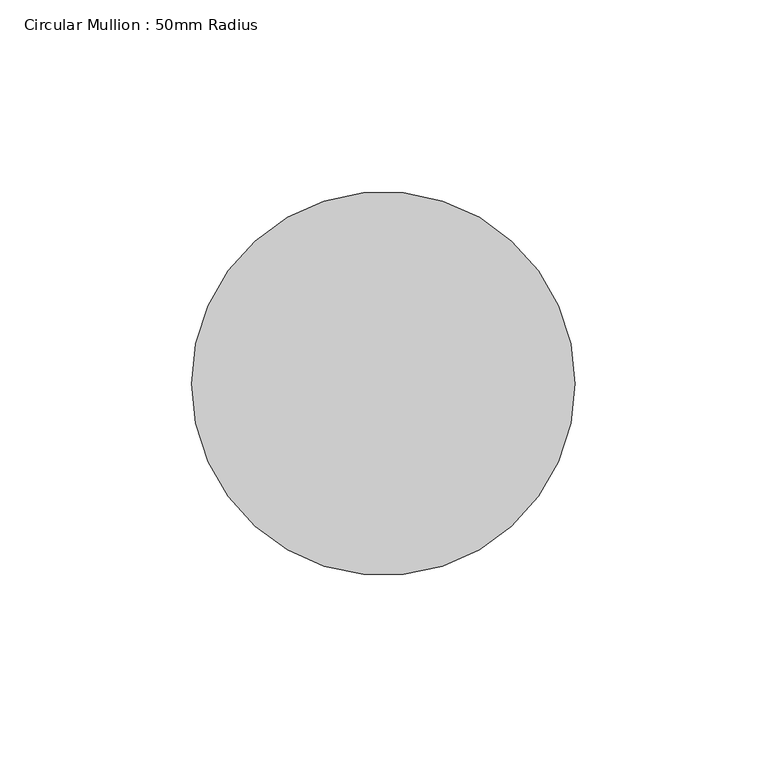
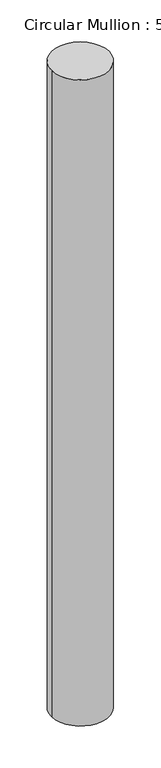
"""IFC4 building model written with IfcOpenShell, lengths in millimetres: member geometry, Circular Mullion : 50mm Radius."""

from ifc_helpers import new_model, si_unit, point, frame, origin, origin_2d, place, context, project, spatial, circle_curve, trimmed, segment, composite_curve, outline, extrude, source, transform, mapped, element, save


def circular_mullion_50mm_radius_da3aa2d7(model_context):
    return source(origin(), model_context, "Body", "SweptSolid", [
        extrude(outline(composite_curve([segment(trimmed(circle_curve(origin_2d(), 50.0), [point((50.0, 0.0))], [point((-50.0, 0.0))], False, "CARTESIAN"), True, "CONTINUOUS"), segment(trimmed(circle_curve(origin_2d(), 50.0), [point((-50.0, 0.0))], [point((50.0, 0.0))], False, "CARTESIAN"), True, "CONTINUOUS")], self_intersect=False)), frame((0.0, 0.0, -1186.6937644), z_axis=(0.0, 0.0, 1.0), x_axis=(1.0, 0.0, 0.0)), (0.0, 0.0, 1.0), 1186.6937644),
    ])


if __name__ == "__main__":
    model = new_model("IFC4")
    model_context = context("Model", 3, world=origin())
    ifc_project = project(units=[si_unit("LENGTHUNIT", "METRE", prefix="MILLI")], contexts=[model_context])
    site = spatial("IfcSite", under=ifc_project)
    building = spatial("IfcBuilding", under=site)
    placement = place(None, origin())
    circular_mullion_50mm_radius_shape = circular_mullion_50mm_radius_da3aa2d7(model_context)
    element("IfcMember", 1, ObjectType="Circular Mullion : 50mm Radius", at=placement, inside=building, context=model_context, shape_type="MappedRepresentation", body=[
        mapped(circular_mullion_50mm_radius_shape, transform((0.0, 0.0, 0.0), x_axis=(1.0, 0.0, 0.0), y_axis=(0.0, 1.0, 0.0), z_axis=(0.0, 0.0, 1.0))),
    ])
    save(model, "model.ifc")

# Revit data of these elements
# Type "Circular Mullion : 50mm Radius"
#   built-in parameter 1007350 = 0.164042 (stored number, unit not read)
# Element 1 (IfcMember, "Circular Mullion : 50mm Radius")
#   Materials on its faces: "Aluminium"
# Materials
#   "Aluminium": class "Metal", colour RGB 247 247 247, transparency 0, Description = "Aluminium 6061", Cost = 0
